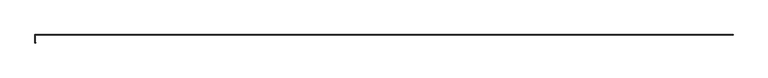
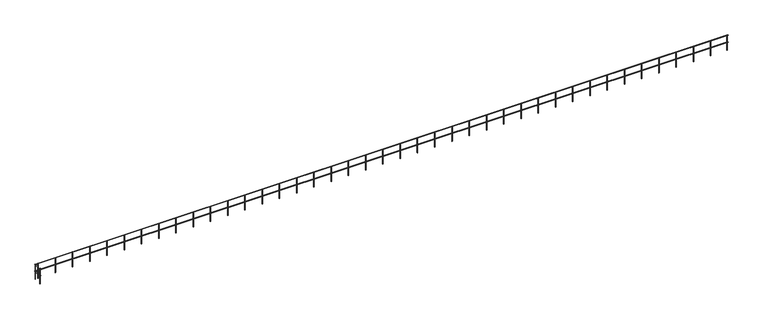
"""IFC4 building model written with IfcOpenShell, lengths in millimetres: railing geometry."""

import ifcopenshell
import ifcopenshell.guid

model = None  # the IFC model being written
_history = None  # IfcOwnerHistory: only IFC2X3 demands one
_inside = {}  # id of a spatial element -> (the spatial element, [elements in it])
_under = {}  # id of a project, library or spatial element -> (it, [spatial elements below it])
_declared = {}  # id of a project -> (the project, [libraries it declares])
_typed = {}  # id of a type object -> (the type object, [elements of that type])
_made_of = {}  # id of a material, layer set ... -> (it, [elements and type objects made of it])


def new_model(schema):
    """Start an empty IFC model of exactly this schema.

    Asked for "IFC4X3", IfcOpenShell would pick the latest addendum, in which some entities
    have other attributes; the version numbers below select the first issue.
    IFC2X3 requires an IfcOwnerHistory on every rooted entity: one is made here for all.
    """
    global model, _history
    if schema == "IFC4X3":
        model = ifcopenshell.file(schema_version=(4, 3, 0, 0))
    else:
        model = ifcopenshell.file(schema=schema)
    _inside.clear()
    _under.clear()
    _declared.clear()
    _typed.clear()
    _made_of.clear()
    _history = None
    if model.schema == "IFC2X3":
        org = make("IfcOrganization", Name="unknown")
        user = make(
            "IfcPersonAndOrganization",
            ThePerson=make("IfcPerson", FamilyName="unknown"),
            TheOrganization=org,
        )
        app = make(
            "IfcApplication",
            ApplicationDeveloper=org,
            Version="unknown",
            ApplicationFullName="unknown",
            ApplicationIdentifier="unknown",
        )
        _history = make(
            "IfcOwnerHistory",
            OwningUser=user,
            OwningApplication=app,
            ChangeAction="ADDED",
            CreationDate=0,
        )
    return model


def make(cls, **values):
    """One entity of the class cls with the attributes given. An attribute that is None is left unset."""
    return model.create_entity(
        cls, **{name: value for name, value in values.items() if value is not None}
    )


def rooted(cls, **values):
    """An entity with a GlobalId (a new one), such as an element, a storey or a relation."""
    return make(cls, GlobalId=ifcopenshell.guid.new(), OwnerHistory=_history, **values)


def si_unit(unit_type, name, prefix=None):
    """IfcSIUnit, for example si_unit("LENGTHUNIT", "METRE", prefix="MILLI")."""
    return make("IfcSIUnit", UnitType=unit_type, Prefix=prefix, Name=name)


def assignment(units):
    """IfcUnitAssignment: the units of a project."""
    return None if units is None else make("IfcUnitAssignment", Units=units)


def point(xyz):
    """IfcCartesianPoint."""
    return None if xyz is None else make("IfcCartesianPoint", Coordinates=xyz)


def direction(xyz):
    """IfcDirection."""
    return None if xyz is None else make("IfcDirection", DirectionRatios=xyz)


def frame(location, z_axis=None, x_axis=None):
    """IfcAxis2Placement3D, a coordinate frame: its origin and axes. An axis left out is left unset."""
    return make(
        "IfcAxis2Placement3D",
        Location=point(location),
        Axis=direction(z_axis),
        RefDirection=direction(x_axis),
    )


def frame_2d(location, x_axis=None):
    """IfcAxis2Placement2D, a coordinate frame in the plane: its origin and x axis."""
    return make(
        "IfcAxis2Placement2D", Location=point(location), RefDirection=direction(x_axis)
    )


def origin():
    """The frame at (0, 0, 0) with its axes left unset."""
    return frame((0.0, 0.0, 0.0))


def place(relative_to, where):
    """IfcLocalPlacement: puts the frame where relative to a parent placement (None: the world)."""
    return make(
        "IfcLocalPlacement", PlacementRelTo=relative_to, RelativePlacement=where
    )


def context(
    kind, dimensions, precision=None, world=None, true_north=None, identifier=None
):
    """IfcGeometricRepresentationContext, for example the 3D "Model" context."""
    return make(
        "IfcGeometricRepresentationContext",
        ContextIdentifier=identifier,
        ContextType=kind,
        CoordinateSpaceDimension=dimensions,
        Precision=precision,
        WorldCoordinateSystem=world,
        TrueNorth=true_north,
    )


def project(units=None, contexts=None):
    """IfcProject with its units and contexts."""
    return rooted(
        "IfcProject",
        Name="project",
        RepresentationContexts=contexts,
        UnitsInContext=assignment(units),
    )


def spatial(cls, under=None, at=None, **own):
    """A site, building, storey or space (cls), placed at a placement, below another one or the project."""
    s = rooted(cls, ObjectPlacement=at, **own)
    if under is not None:
        _under.setdefault(under.id(), (under, []))[1].append(s)
    return s


def circle_curve(where, radius):
    """IfcCircle in the frame where."""
    return make("IfcCircle", Position=where, Radius=radius)


def ellipse_curve(where, semi_axis1, semi_axis2):
    """IfcEllipse in the frame where."""
    return make(
        "IfcEllipse", Position=where, SemiAxis1=semi_axis1, SemiAxis2=semi_axis2
    )


def trimmed(basis, trim1, trim2, sense, master):
    """IfcTrimmedCurve: the piece of a basis curve between two trims."""
    return make(
        "IfcTrimmedCurve",
        BasisCurve=basis,
        Trim1=trim1,
        Trim2=trim2,
        SenseAgreement=sense,
        MasterRepresentation=master,
    )


def segment(curve, same_sense, transition):
    """IfcCompositeCurveSegment."""
    return make(
        "IfcCompositeCurveSegment",
        Transition=transition,
        SameSense=same_sense,
        ParentCurve=curve,
    )


def composite_curve(segments, self_intersect=None):
    """IfcCompositeCurve: segments joined end to end."""
    return make("IfcCompositeCurve", Segments=segments, SelfIntersect=self_intersect)


def outline(outer, holes=None, kind="AREA"):
    """IfcArbitraryClosedProfileDef: a profile drawn as a closed curve; with holes, ...WithVoids."""
    if holes is None:
        return make("IfcArbitraryClosedProfileDef", ProfileType=kind, OuterCurve=outer)
    return make(
        "IfcArbitraryProfileDefWithVoids",
        ProfileType=kind,
        OuterCurve=outer,
        InnerCurves=holes,
    )


def extrude(swept, where, along, depth):
    """IfcExtrudedAreaSolid: the profile swept, set in the frame where, extruded along a direction by depth."""
    return make(
        "IfcExtrudedAreaSolid",
        SweptArea=swept,
        Position=where,
        ExtrudedDirection=direction(along),
        Depth=depth,
    )


def shape(context_of_items, identifier, shape_type, items):
    """IfcShapeRepresentation: the items that make up one representation, for example the "Body"."""
    return make(
        "IfcShapeRepresentation",
        ContextOfItems=context_of_items,
        RepresentationIdentifier=identifier,
        RepresentationType=shape_type,
        Items=items,
    )


def source(mapping_origin, context_of_items, identifier, shape_type, items):
    """IfcRepresentationMap: a shape defined once, which mapped items show again and again."""
    return make(
        "IfcRepresentationMap",
        MappingOrigin=mapping_origin,
        MappedRepresentation=shape(context_of_items, identifier, shape_type, items),
    )


def transform(
    local_origin,
    x_axis=None,
    y_axis=None,
    z_axis=None,
    scale=None,
    scale2=None,
    scale3=None,
    uniform=True,
):
    """IfcCartesianTransformationOperator3D, or its non-uniform kind. x_axis, y_axis, z_axis: its Axis1, 2, 3."""
    if uniform:
        return make(
            "IfcCartesianTransformationOperator3D",
            Axis1=direction(x_axis),
            Axis2=direction(y_axis),
            LocalOrigin=point(local_origin),
            Scale=scale,
            Axis3=direction(z_axis),
        )
    return make(
        "IfcCartesianTransformationOperator3DnonUniform",
        Axis1=direction(x_axis),
        Axis2=direction(y_axis),
        LocalOrigin=point(local_origin),
        Scale=scale,
        Axis3=direction(z_axis),
        Scale2=scale2,
        Scale3=scale3,
    )


def mapped(mapping_source, mapping_target):
    """IfcMappedItem: shows the shape of a source again, moved by a transform."""
    return make(
        "IfcMappedItem", MappingSource=mapping_source, MappingTarget=mapping_target
    )


def made_of(thing, what):
    """Note that an element or type object is made of a material, layer set ...; save() writes the relation."""
    if what is not None:
        _made_of.setdefault(what.id(), (what, []))[1].append(thing)
    return thing


def element(
    cls,
    number,
    at=None,
    inside=None,
    cuts=None,
    type_object=None,
    material=None,
    context=None,
    identifier="Body",
    shape_type=None,
    held_by="IfcProductDefinitionShape",
    body=None,
    shapes=None,
    **own,
):
    """One element of the class cls, such as IfcWall. Its Tag is "e" and its number.

    at: its placement. inside: the storey or other place that contains it. cuts: it is an
    opening in that element (IfcRelVoidsElement). A single representation is given by context,
    identifier, shape_type and body (its items); several are given by shapes. held_by: the class
    of the entity that holds the representations. save() writes the other relations.
    """
    e = rooted(cls, Tag="e%d" % number, ObjectPlacement=at, **own)
    if body is not None:
        shapes = [shape(context, identifier, shape_type, body)]
    if shapes is not None:
        e.Representation = make(held_by, Representations=shapes)
    if inside is not None:
        _inside.setdefault(inside.id(), (inside, []))[1].append(e)
    if cuts is not None:
        rooted(
            "IfcRelVoidsElement", RelatingBuildingElement=cuts, RelatedOpeningElement=e
        )
    if type_object is not None:
        _typed.setdefault(type_object.id(), (type_object, []))[1].append(e)
    return made_of(e, material)


def aggregate(whole, parts):
    """IfcRelAggregates: a whole, such as a stair, and the parts it consists of."""
    return rooted("IfcRelAggregates", RelatingObject=whole, RelatedObjects=parts)


def save(model, path):
    """Write the relations noted so far, then the file.

    IfcRelAggregates (storeys below a building ...), IfcRelContainedInSpatialStructure (elements
    in a storey), IfcRelDefinesByType, IfcRelAssociatesMaterial and IfcRelDeclares: one each for
    every whole, place, type object, material and project.
    """
    for whole, parts in _under.values():
        aggregate(whole, parts)
    for where, things in _inside.values():
        rooted(
            "IfcRelContainedInSpatialStructure",
            RelatedElements=things,
            RelatingStructure=where,
        )
    for kind, things in _typed.values():
        rooted("IfcRelDefinesByType", RelatedObjects=things, RelatingType=kind)
    for what, things in _made_of.values():
        rooted("IfcRelAssociatesMaterial", RelatedObjects=things, RelatingMaterial=what)
    for by, libraries in _declared.values():
        rooted("IfcRelDeclares", RelatingContext=by, RelatedDefinitions=libraries)
    model.write(path)


def plane_surface(at):
    """IfcPlane: the flat surface through the origin of the frame at, square to its z axis."""
    return make("IfcPlane", Position=at)


def cylinder_surface(at, radius):
    """IfcCylindricalSurface: all points at the distance radius from the z axis of the frame at."""
    return make("IfcCylindricalSurface", Position=at, Radius=radius)


def advanced_brep(points, edges, surfaces, faces):
    """IfcAdvancedBrep: a solid bounded by faces that lie on surfaces and meet in shared edges.

    An edge is (start, end): straight between two places in points (the first is 0);
    or (start, end, curve); or (start, end, curve, False) where it runs against its curve.
    A face is (place in surfaces, loops), or (place, loops, False) where it looks against
    its surface's normal. A loop lists edges by number (the first is 1), with a minus sign
    where the edge is run from its end to its start. The first loop is the outer one.
    """
    corners = [point(p) for p in points]
    vertices = [make("IfcVertexPoint", VertexGeometry=c) for c in corners]
    made = []
    for start, end, *more in edges:
        made.append(
            make(
                "IfcEdgeCurve",
                EdgeStart=vertices[start],
                EdgeEnd=vertices[end],
                EdgeGeometry=more[0] if more else make("IfcPolyline", Points=[corners[start], corners[end]]),
                SameSense=more[1] if len(more) > 1 else True,
            )
        )
    hull = []
    for where, loops, *sense in faces:
        bounds = []
        for j, loop in enumerate(loops):
            ring = [make("IfcOrientedEdge", EdgeElement=made[abs(k) - 1], Orientation=k > 0) for k in loop]
            bounds.append(
                make(
                    "IfcFaceOuterBound" if j == 0 else "IfcFaceBound",
                    Bound=make("IfcEdgeLoop", EdgeList=ring),
                    Orientation=True,
                )
            )
        hull.append(make("IfcAdvancedFace", Bounds=bounds, FaceSurface=surfaces[where], SameSense=sense[0] if sense else True))
    return make("IfcAdvancedBrep", Outer=make("IfcClosedShell", CfsFaces=hull))


def railing_e0085468(model_context):
    return source(origin(), model_context, "Body", "SolidModel", [
        advanced_brep(
        [(74181.0, -4167.9791411, 885.0), (74181.0, -4137.9791411, 885.0), (26002.0, -4167.9791411, 885.0), (25972.0, -4137.9791411, 885.0), (26002.0, -4687.9791411, 885.0), (25972.0, -4717.9791411, 885.0), (26040.0, -4687.9791411, 885.0), (26040.0, -4717.9791411, 885.0)],
        [
            (0, 1, circle_curve(frame((74181.0, -4152.9791411, 885.0), z_axis=(1.0, 0.0, 0.0), x_axis=(0.0, 1.0, 0.0)), 15.0)),
            (1, 0, circle_curve(frame((74181.0, -4152.9791411, 885.0), z_axis=(1.0, 0.0, 0.0), x_axis=(0.0, 1.0, 0.0)), 15.0)),
            (0, 2),
            (2, 3, ellipse_curve(frame((25987.0, -4152.9791411, 885.0), z_axis=(0.7071067811865487, 0.7071067811865464, 0.0), x_axis=(0.7071067811865465, -0.7071067811865487, 0.0)), 21.2132034, 15.0)),
            (3, 1),
            (3, 2, ellipse_curve(frame((25987.0, -4152.9791411, 885.0), z_axis=(0.7071067811865487, 0.7071067811865464, 0.0), x_axis=(0.7071067811865465, -0.7071067811865487, 0.0)), 21.2132034, 15.0)),
            (2, 4),
            (4, 5, ellipse_curve(frame((25987.0, -4702.9791411, 885.0), z_axis=(-0.7071067811865475, 0.7071067811865475, 0.0), x_axis=(0.7071067811865474, 0.7071067811865476, 0.0)), 21.2132034, 15.0)),
            (5, 3),
            (5, 4, ellipse_curve(frame((25987.0, -4702.9791411, 885.0), z_axis=(-0.7071067811865475, 0.7071067811865475, 0.0), x_axis=(0.7071067811865474, 0.7071067811865476, 0.0)), 21.2132034, 15.0)),
            (6, 7, circle_curve(frame((26040.0, -4702.9791411, 885.0), z_axis=(1.0, 0.0, 0.0), x_axis=(0.0, -1.0, 0.0)), 15.0)),
            (7, 6, circle_curve(frame((26040.0, -4702.9791411, 885.0), z_axis=(1.0, 0.0, 0.0), x_axis=(0.0, -1.0, 0.0)), 15.0)),
            (4, 6),
            (7, 5),
        ],
        [
            plane_surface(frame((74181.0, -4152.9791411, 900.0), z_axis=(1.0, 0.0, 0.0), x_axis=(0.0, -1.0, 0.0))),
            cylinder_surface(frame((74181.0, -4152.9791411, 885.0), z_axis=(1.0, 0.0, 0.0), x_axis=(0.0, 1.0, 0.0)), 15.0),
            cylinder_surface(frame((25987.0, -4152.9791411, 885.0), z_axis=(0.0, 1.0, 0.0), x_axis=(-1.0, 0.0, 0.0)), 15.0),
            plane_surface(frame((26040.0, -4702.9791411, 900.0), z_axis=(1.0, 0.0, 0.0), x_axis=(0.0, 1.0, 0.0))),
            cylinder_surface(frame((25987.0, -4702.9791411, 885.0), z_axis=(-1.0, 0.0, 0.0), x_axis=(0.0, -1.0, 0.0)), 15.0),
        ],
        [
            (0, [[1, 2]]),
            (1, [[-1, 3, 4, 5]]),
            (1, [[-2, -5, 6, -3]]),
            (2, [[-4, 7, 8, 9]]),
            (2, [[-6, -9, 10, -7]]),
            (3, [[11, 12]]),
            (4, [[-8, 13, -12, 14]]),
            (4, [[-10, -14, -11, -13]]),
        ],
    ),
        advanced_brep(
        [(74181.0, -4167.9791411, 1385.0), (74181.0, -4137.9791411, 1385.0), (26002.0, -4167.9791411, 1385.0), (25972.0, -4137.9791411, 1385.0), (26002.0, -4687.9791411, 1385.0), (25972.0, -4717.9791411, 1385.0), (26040.0, -4687.9791411, 1385.0), (26040.0, -4717.9791411, 1385.0)],
        [
            (0, 1, circle_curve(frame((74181.0, -4152.9791411, 1385.0), z_axis=(1.0, 0.0, 0.0), x_axis=(0.0, 1.0, 0.0)), 15.0)),
            (1, 0, circle_curve(frame((74181.0, -4152.9791411, 1385.0), z_axis=(1.0, 0.0, 0.0), x_axis=(0.0, 1.0, 0.0)), 15.0)),
            (0, 2),
            (2, 3, ellipse_curve(frame((25987.0, -4152.9791411, 1385.0), z_axis=(0.7071067811865487, 0.7071067811865464, 0.0), x_axis=(0.7071067811865465, -0.7071067811865487, 0.0)), 21.2132034, 15.0)),
            (3, 1),
            (3, 2, ellipse_curve(frame((25987.0, -4152.9791411, 1385.0), z_axis=(0.7071067811865487, 0.7071067811865464, 0.0), x_axis=(0.7071067811865465, -0.7071067811865487, 0.0)), 21.2132034, 15.0)),
            (2, 4),
            (4, 5, ellipse_curve(frame((25987.0, -4702.9791411, 1385.0), z_axis=(-0.7071067811865475, 0.7071067811865475, 0.0), x_axis=(0.7071067811865474, 0.7071067811865476, 0.0)), 21.2132034, 15.0)),
            (5, 3),
            (5, 4, ellipse_curve(frame((25987.0, -4702.9791411, 1385.0), z_axis=(-0.7071067811865475, 0.7071067811865475, 0.0), x_axis=(0.7071067811865474, 0.7071067811865476, 0.0)), 21.2132034, 15.0)),
            (6, 7, circle_curve(frame((26040.0, -4702.9791411, 1385.0), z_axis=(1.0, 0.0, 0.0), x_axis=(0.0, -1.0, 0.0)), 15.0)),
            (7, 6, circle_curve(frame((26040.0, -4702.9791411, 1385.0), z_axis=(1.0, 0.0, 0.0), x_axis=(0.0, -1.0, 0.0)), 15.0)),
            (4, 6),
            (7, 5),
        ],
        [
            plane_surface(frame((74181.0, -4152.9791411, 1400.0), z_axis=(1.0, 0.0, 0.0), x_axis=(0.0, -1.0, 0.0))),
            cylinder_surface(frame((74181.0, -4152.9791411, 1385.0), z_axis=(1.0, 0.0, 0.0), x_axis=(0.0, 1.0, 0.0)), 15.0),
            cylinder_surface(frame((25987.0, -4152.9791411, 1385.0), z_axis=(0.0, 1.0, 0.0), x_axis=(-1.0, 0.0, 0.0)), 15.0),
            plane_surface(frame((26040.0, -4702.9791411, 1400.0), z_axis=(1.0, 0.0, 0.0), x_axis=(0.0, 1.0, 0.0))),
            cylinder_surface(frame((25987.0, -4702.9791411, 1385.0), z_axis=(-1.0, 0.0, 0.0), x_axis=(0.0, -1.0, 0.0)), 15.0),
        ],
        [
            (0, [[1, 2]]),
            (1, [[-1, 3, 4, 5]]),
            (1, [[-2, -5, 6, -3]]),
            (2, [[-4, 7, 8, 9]]),
            (2, [[-6, -9, 10, -7]]),
            (3, [[11, 12]]),
            (4, [[-8, 13, -12, 14]]),
            (4, [[-10, -14, -11, -13]]),
        ],
    ),
        extrude(outline(composite_curve([segment(trimmed(circle_curve(frame_2d((26181.0, -4152.9791411)), 15.0), [point((26181.0, -4167.9791411))], [point((26181.0, -4137.9791411))], False, "CARTESIAN"), True, "CONTINUOUS"), segment(trimmed(circle_curve(frame_2d((26181.0, -4152.9791411)), 15.0), [point((26181.0, -4137.9791411))], [point((26181.0, -4167.9791411))], False, "CARTESIAN"), True, "CONTINUOUS")], self_intersect=False)), frame((0.0, 0.0, 300.0), z_axis=(0.0, 0.0, 1.0), x_axis=(1.0, 0.0, 0.0)), (0.0, 0.0, 1.0), 1070.0),
        extrude(outline(composite_curve([segment(trimmed(circle_curve(frame_2d((27381.0, -4152.9791411)), 15.0), [point((27381.0, -4167.9791411))], [point((27381.0, -4137.9791411))], False, "CARTESIAN"), True, "CONTINUOUS"), segment(trimmed(circle_curve(frame_2d((27381.0, -4152.9791411)), 15.0), [point((27381.0, -4137.9791411))], [point((27381.0, -4167.9791411))], False, "CARTESIAN"), True, "CONTINUOUS")], self_intersect=False)), frame((0.0, 0.0, 300.0), z_axis=(0.0, 0.0, 1.0), x_axis=(1.0, 0.0, 0.0)), (0.0, 0.0, 1.0), 1070.0),
        extrude(outline(composite_curve([segment(trimmed(circle_curve(frame_2d((28581.0, -4152.9791411)), 15.0), [point((28581.0, -4167.9791411))], [point((28581.0, -4137.9791411))], False, "CARTESIAN"), True, "CONTINUOUS"), segment(trimmed(circle_curve(frame_2d((28581.0, -4152.9791411)), 15.0), [point((28581.0, -4137.9791411))], [point((28581.0, -4167.9791411))], False, "CARTESIAN"), True, "CONTINUOUS")], self_intersect=False)), frame((0.0, 0.0, 300.0), z_axis=(0.0, 0.0, 1.0), x_axis=(1.0, 0.0, 0.0)), (0.0, 0.0, 1.0), 1070.0),
        extrude(outline(composite_curve([segment(trimmed(circle_curve(frame_2d((29781.0, -4152.9791411)), 15.0), [point((29781.0, -4167.9791411))], [point((29781.0, -4137.9791411))], False, "CARTESIAN"), True, "CONTINUOUS"), segment(trimmed(circle_curve(frame_2d((29781.0, -4152.9791411)), 15.0), [point((29781.0, -4137.9791411))], [point((29781.0, -4167.9791411))], False, "CARTESIAN"), True, "CONTINUOUS")], self_intersect=False)), frame((0.0, 0.0, 300.0), z_axis=(0.0, 0.0, 1.0), x_axis=(1.0, 0.0, 0.0)), (0.0, 0.0, 1.0), 1070.0),
        extrude(outline(composite_curve([segment(trimmed(circle_curve(frame_2d((30981.0, -4152.9791411)), 15.0), [point((30981.0, -4167.9791411))], [point((30981.0, -4137.9791411))], False, "CARTESIAN"), True, "CONTINUOUS"), segment(trimmed(circle_curve(frame_2d((30981.0, -4152.9791411)), 15.0), [point((30981.0, -4137.9791411))], [point((30981.0, -4167.9791411))], False, "CARTESIAN"), True, "CONTINUOUS")], self_intersect=False)), frame((0.0, 0.0, 300.0), z_axis=(0.0, 0.0, 1.0), x_axis=(1.0, 0.0, 0.0)), (0.0, 0.0, 1.0), 1070.0),
        extrude(outline(composite_curve([segment(trimmed(circle_curve(frame_2d((32181.0, -4152.9791411)), 15.0), [point((32181.0, -4167.9791411))], [point((32181.0, -4137.9791411))], False, "CARTESIAN"), True, "CONTINUOUS"), segment(trimmed(circle_curve(frame_2d((32181.0, -4152.9791411)), 15.0), [point((32181.0, -4137.9791411))], [point((32181.0, -4167.9791411))], False, "CARTESIAN"), True, "CONTINUOUS")], self_intersect=False)), frame((0.0, 0.0, 300.0), z_axis=(0.0, 0.0, 1.0), x_axis=(1.0, 0.0, 0.0)), (0.0, 0.0, 1.0), 1070.0),
        extrude(outline(composite_curve([segment(trimmed(circle_curve(frame_2d((33381.0, -4152.9791411)), 15.0), [point((33381.0, -4167.9791411))], [point((33381.0, -4137.9791411))], False, "CARTESIAN"), True, "CONTINUOUS"), segment(trimmed(circle_curve(frame_2d((33381.0, -4152.9791411)), 15.0), [point((33381.0, -4137.9791411))], [point((33381.0, -4167.9791411))], False, "CARTESIAN"), True, "CONTINUOUS")], self_intersect=False)), frame((0.0, 0.0, 300.0), z_axis=(0.0, 0.0, 1.0), x_axis=(1.0, 0.0, 0.0)), (0.0, 0.0, 1.0), 1070.0),
        extrude(outline(composite_curve([segment(trimmed(circle_curve(frame_2d((34581.0, -4152.9791411)), 15.0), [point((34581.0, -4167.9791411))], [point((34581.0, -4137.9791411))], False, "CARTESIAN"), True, "CONTINUOUS"), segment(trimmed(circle_curve(frame_2d((34581.0, -4152.9791411)), 15.0), [point((34581.0, -4137.9791411))], [point((34581.0, -4167.9791411))], False, "CARTESIAN"), True, "CONTINUOUS")], self_intersect=False)), frame((0.0, 0.0, 300.0), z_axis=(0.0, 0.0, 1.0), x_axis=(1.0, 0.0, 0.0)), (0.0, 0.0, 1.0), 1070.0),
        extrude(outline(composite_curve([segment(trimmed(circle_curve(frame_2d((35781.0, -4152.9791411)), 15.0), [point((35781.0, -4167.9791411))], [point((35781.0, -4137.9791411))], False, "CARTESIAN"), True, "CONTINUOUS"), segment(trimmed(circle_curve(frame_2d((35781.0, -4152.9791411)), 15.0), [point((35781.0, -4137.9791411))], [point((35781.0, -4167.9791411))], False, "CARTESIAN"), True, "CONTINUOUS")], self_intersect=False)), frame((0.0, 0.0, 300.0), z_axis=(0.0, 0.0, 1.0), x_axis=(1.0, 0.0, 0.0)), (0.0, 0.0, 1.0), 1070.0),
        extrude(outline(composite_curve([segment(trimmed(circle_curve(frame_2d((36981.0, -4152.9791411)), 15.0), [point((36981.0, -4167.9791411))], [point((36981.0, -4137.9791411))], False, "CARTESIAN"), True, "CONTINUOUS"), segment(trimmed(circle_curve(frame_2d((36981.0, -4152.9791411)), 15.0), [point((36981.0, -4137.9791411))], [point((36981.0, -4167.9791411))], False, "CARTESIAN"), True, "CONTINUOUS")], self_intersect=False)), frame((0.0, 0.0, 300.0), z_axis=(0.0, 0.0, 1.0), x_axis=(1.0, 0.0, 0.0)), (0.0, 0.0, 1.0), 1070.0),
        extrude(outline(composite_curve([segment(trimmed(circle_curve(frame_2d((38181.0, -4152.9791411)), 15.0), [point((38181.0, -4167.9791411))], [point((38181.0, -4137.9791411))], False, "CARTESIAN"), True, "CONTINUOUS"), segment(trimmed(circle_curve(frame_2d((38181.0, -4152.9791411)), 15.0), [point((38181.0, -4137.9791411))], [point((38181.0, -4167.9791411))], False, "CARTESIAN"), True, "CONTINUOUS")], self_intersect=False)), frame((0.0, 0.0, 300.0), z_axis=(0.0, 0.0, 1.0), x_axis=(1.0, 0.0, 0.0)), (0.0, 0.0, 1.0), 1070.0),
        extrude(outline(composite_curve([segment(trimmed(circle_curve(frame_2d((39381.0, -4152.9791411)), 15.0), [point((39381.0, -4167.9791411))], [point((39381.0, -4137.9791411))], False, "CARTESIAN"), True, "CONTINUOUS"), segment(trimmed(circle_curve(frame_2d((39381.0, -4152.9791411)), 15.0), [point((39381.0, -4137.9791411))], [point((39381.0, -4167.9791411))], False, "CARTESIAN"), True, "CONTINUOUS")], self_intersect=False)), frame((0.0, 0.0, 300.0), z_axis=(0.0, 0.0, 1.0), x_axis=(1.0, 0.0, 0.0)), (0.0, 0.0, 1.0), 1070.0),
        extrude(outline(composite_curve([segment(trimmed(circle_curve(frame_2d((40581.0, -4152.9791411)), 15.0), [point((40581.0, -4167.9791411))], [point((40581.0, -4137.9791411))], False, "CARTESIAN"), True, "CONTINUOUS"), segment(trimmed(circle_curve(frame_2d((40581.0, -4152.9791411)), 15.0), [point((40581.0, -4137.9791411))], [point((40581.0, -4167.9791411))], False, "CARTESIAN"), True, "CONTINUOUS")], self_intersect=False)), frame((0.0, 0.0, 300.0), z_axis=(0.0, 0.0, 1.0), x_axis=(1.0, 0.0, 0.0)), (0.0, 0.0, 1.0), 1070.0),
        extrude(outline(composite_curve([segment(trimmed(circle_curve(frame_2d((41781.0, -4152.9791411)), 15.0), [point((41781.0, -4167.9791411))], [point((41781.0, -4137.9791411))], False, "CARTESIAN"), True, "CONTINUOUS"), segment(trimmed(circle_curve(frame_2d((41781.0, -4152.9791411)), 15.0), [point((41781.0, -4137.9791411))], [point((41781.0, -4167.9791411))], False, "CARTESIAN"), True, "CONTINUOUS")], self_intersect=False)), frame((0.0, 0.0, 300.0), z_axis=(0.0, 0.0, 1.0), x_axis=(1.0, 0.0, 0.0)), (0.0, 0.0, 1.0), 1070.0),
        extrude(outline(composite_curve([segment(trimmed(circle_curve(frame_2d((42981.0, -4152.9791411)), 15.0), [point((42981.0, -4167.9791411))], [point((42981.0, -4137.9791411))], False, "CARTESIAN"), True, "CONTINUOUS"), segment(trimmed(circle_curve(frame_2d((42981.0, -4152.9791411)), 15.0), [point((42981.0, -4137.9791411))], [point((42981.0, -4167.9791411))], False, "CARTESIAN"), True, "CONTINUOUS")], self_intersect=False)), frame((0.0, 0.0, 300.0), z_axis=(0.0, 0.0, 1.0), x_axis=(1.0, 0.0, 0.0)), (0.0, 0.0, 1.0), 1070.0),
        extrude(outline(composite_curve([segment(trimmed(circle_curve(frame_2d((44181.0, -4152.9791411)), 15.0), [point((44181.0, -4167.9791411))], [point((44181.0, -4137.9791411))], False, "CARTESIAN"), True, "CONTINUOUS"), segment(trimmed(circle_curve(frame_2d((44181.0, -4152.9791411)), 15.0), [point((44181.0, -4137.9791411))], [point((44181.0, -4167.9791411))], False, "CARTESIAN"), True, "CONTINUOUS")], self_intersect=False)), frame((0.0, 0.0, 300.0), z_axis=(0.0, 0.0, 1.0), x_axis=(1.0, 0.0, 0.0)), (0.0, 0.0, 1.0), 1070.0),
        extrude(outline(composite_curve([segment(trimmed(circle_curve(frame_2d((45381.0, -4152.9791411)), 15.0), [point((45381.0, -4167.9791411))], [point((45381.0, -4137.9791411))], False, "CARTESIAN"), True, "CONTINUOUS"), segment(trimmed(circle_curve(frame_2d((45381.0, -4152.9791411)), 15.0), [point((45381.0, -4137.9791411))], [point((45381.0, -4167.9791411))], False, "CARTESIAN"), True, "CONTINUOUS")], self_intersect=False)), frame((0.0, 0.0, 300.0), z_axis=(0.0, 0.0, 1.0), x_axis=(1.0, 0.0, 0.0)), (0.0, 0.0, 1.0), 1070.0),
        extrude(outline(composite_curve([segment(trimmed(circle_curve(frame_2d((46581.0, -4152.9791411)), 15.0), [point((46581.0, -4167.9791411))], [point((46581.0, -4137.9791411))], False, "CARTESIAN"), True, "CONTINUOUS"), segment(trimmed(circle_curve(frame_2d((46581.0, -4152.9791411)), 15.0), [point((46581.0, -4137.9791411))], [point((46581.0, -4167.9791411))], False, "CARTESIAN"), True, "CONTINUOUS")], self_intersect=False)), frame((0.0, 0.0, 300.0), z_axis=(0.0, 0.0, 1.0), x_axis=(1.0, 0.0, 0.0)), (0.0, 0.0, 1.0), 1070.0),
        extrude(outline(composite_curve([segment(trimmed(circle_curve(frame_2d((47781.0, -4152.9791411)), 15.0), [point((47781.0, -4167.9791411))], [point((47781.0, -4137.9791411))], False, "CARTESIAN"), True, "CONTINUOUS"), segment(trimmed(circle_curve(frame_2d((47781.0, -4152.9791411)), 15.0), [point((47781.0, -4137.9791411))], [point((47781.0, -4167.9791411))], False, "CARTESIAN"), True, "CONTINUOUS")], self_intersect=False)), frame((0.0, 0.0, 300.0), z_axis=(0.0, 0.0, 1.0), x_axis=(1.0, 0.0, 0.0)), (0.0, 0.0, 1.0), 1070.0),
        extrude(outline(composite_curve([segment(trimmed(circle_curve(frame_2d((48981.0, -4152.9791411)), 15.0), [point((48981.0, -4167.9791411))], [point((48981.0, -4137.9791411))], False, "CARTESIAN"), True, "CONTINUOUS"), segment(trimmed(circle_curve(frame_2d((48981.0, -4152.9791411)), 15.0), [point((48981.0, -4137.9791411))], [point((48981.0, -4167.9791411))], False, "CARTESIAN"), True, "CONTINUOUS")], self_intersect=False)), frame((0.0, 0.0, 300.0), z_axis=(0.0, 0.0, 1.0), x_axis=(1.0, 0.0, 0.0)), (0.0, 0.0, 1.0), 1070.0),
        extrude(outline(composite_curve([segment(trimmed(circle_curve(frame_2d((50181.0, -4152.9791411)), 15.0), [point((50181.0, -4167.9791411))], [point((50181.0, -4137.9791411))], False, "CARTESIAN"), True, "CONTINUOUS"), segment(trimmed(circle_curve(frame_2d((50181.0, -4152.9791411)), 15.0), [point((50181.0, -4137.9791411))], [point((50181.0, -4167.9791411))], False, "CARTESIAN"), True, "CONTINUOUS")], self_intersect=False)), frame((0.0, 0.0, 300.0), z_axis=(0.0, 0.0, 1.0), x_axis=(1.0, 0.0, 0.0)), (0.0, 0.0, 1.0), 1070.0),
        extrude(outline(composite_curve([segment(trimmed(circle_curve(frame_2d((51381.0, -4152.9791411)), 15.0), [point((51381.0, -4167.9791411))], [point((51381.0, -4137.9791411))], False, "CARTESIAN"), True, "CONTINUOUS"), segment(trimmed(circle_curve(frame_2d((51381.0, -4152.9791411)), 15.0), [point((51381.0, -4137.9791411))], [point((51381.0, -4167.9791411))], False, "CARTESIAN"), True, "CONTINUOUS")], self_intersect=False)), frame((0.0, 0.0, 300.0), z_axis=(0.0, 0.0, 1.0), x_axis=(1.0, 0.0, 0.0)), (0.0, 0.0, 1.0), 1070.0),
        extrude(outline(composite_curve([segment(trimmed(circle_curve(frame_2d((52581.0, -4152.9791411)), 15.0), [point((52581.0, -4167.9791411))], [point((52581.0, -4137.9791411))], False, "CARTESIAN"), True, "CONTINUOUS"), segment(trimmed(circle_curve(frame_2d((52581.0, -4152.9791411)), 15.0), [point((52581.0, -4137.9791411))], [point((52581.0, -4167.9791411))], False, "CARTESIAN"), True, "CONTINUOUS")], self_intersect=False)), frame((0.0, 0.0, 300.0), z_axis=(0.0, 0.0, 1.0), x_axis=(1.0, 0.0, 0.0)), (0.0, 0.0, 1.0), 1070.0),
        extrude(outline(composite_curve([segment(trimmed(circle_curve(frame_2d((53781.0, -4152.9791411)), 15.0), [point((53781.0, -4167.9791411))], [point((53781.0, -4137.9791411))], False, "CARTESIAN"), True, "CONTINUOUS"), segment(trimmed(circle_curve(frame_2d((53781.0, -4152.9791411)), 15.0), [point((53781.0, -4137.9791411))], [point((53781.0, -4167.9791411))], False, "CARTESIAN"), True, "CONTINUOUS")], self_intersect=False)), frame((0.0, 0.0, 300.0), z_axis=(0.0, 0.0, 1.0), x_axis=(1.0, 0.0, 0.0)), (0.0, 0.0, 1.0), 1070.0),
        extrude(outline(composite_curve([segment(trimmed(circle_curve(frame_2d((54981.0, -4152.9791411)), 15.0), [point((54981.0, -4167.9791411))], [point((54981.0, -4137.9791411))], False, "CARTESIAN"), True, "CONTINUOUS"), segment(trimmed(circle_curve(frame_2d((54981.0, -4152.9791411)), 15.0), [point((54981.0, -4137.9791411))], [point((54981.0, -4167.9791411))], False, "CARTESIAN"), True, "CONTINUOUS")], self_intersect=False)), frame((0.0, 0.0, 300.0), z_axis=(0.0, 0.0, 1.0), x_axis=(1.0, 0.0, 0.0)), (0.0, 0.0, 1.0), 1070.0),
        extrude(outline(composite_curve([segment(trimmed(circle_curve(frame_2d((56181.0, -4152.9791411)), 15.0), [point((56181.0, -4167.9791411))], [point((56181.0, -4137.9791411))], False, "CARTESIAN"), True, "CONTINUOUS"), segment(trimmed(circle_curve(frame_2d((56181.0, -4152.9791411)), 15.0), [point((56181.0, -4137.9791411))], [point((56181.0, -4167.9791411))], False, "CARTESIAN"), True, "CONTINUOUS")], self_intersect=False)), frame((0.0, 0.0, 300.0), z_axis=(0.0, 0.0, 1.0), x_axis=(1.0, 0.0, 0.0)), (0.0, 0.0, 1.0), 1070.0),
        extrude(outline(composite_curve([segment(trimmed(circle_curve(frame_2d((57381.0, -4152.9791411)), 15.0), [point((57381.0, -4167.9791411))], [point((57381.0, -4137.9791411))], False, "CARTESIAN"), True, "CONTINUOUS"), segment(trimmed(circle_curve(frame_2d((57381.0, -4152.9791411)), 15.0), [point((57381.0, -4137.9791411))], [point((57381.0, -4167.9791411))], False, "CARTESIAN"), True, "CONTINUOUS")], self_intersect=False)), frame((0.0, 0.0, 300.0), z_axis=(0.0, 0.0, 1.0), x_axis=(1.0, 0.0, 0.0)), (0.0, 0.0, 1.0), 1070.0),
        extrude(outline(composite_curve([segment(trimmed(circle_curve(frame_2d((58581.0, -4152.9791411)), 15.0), [point((58581.0, -4167.9791411))], [point((58581.0, -4137.9791411))], False, "CARTESIAN"), True, "CONTINUOUS"), segment(trimmed(circle_curve(frame_2d((58581.0, -4152.9791411)), 15.0), [point((58581.0, -4137.9791411))], [point((58581.0, -4167.9791411))], False, "CARTESIAN"), True, "CONTINUOUS")], self_intersect=False)), frame((0.0, 0.0, 300.0), z_axis=(0.0, 0.0, 1.0), x_axis=(1.0, 0.0, 0.0)), (0.0, 0.0, 1.0), 1070.0),
        extrude(outline(composite_curve([segment(trimmed(circle_curve(frame_2d((59781.0, -4152.9791411)), 15.0), [point((59781.0, -4167.9791411))], [point((59781.0, -4137.9791411))], False, "CARTESIAN"), True, "CONTINUOUS"), segment(trimmed(circle_curve(frame_2d((59781.0, -4152.9791411)), 15.0), [point((59781.0, -4137.9791411))], [point((59781.0, -4167.9791411))], False, "CARTESIAN"), True, "CONTINUOUS")], self_intersect=False)), frame((0.0, 0.0, 300.0), z_axis=(0.0, 0.0, 1.0), x_axis=(1.0, 0.0, 0.0)), (0.0, 0.0, 1.0), 1070.0),
        extrude(outline(composite_curve([segment(trimmed(circle_curve(frame_2d((60981.0, -4152.9791411)), 15.0), [point((60981.0, -4167.9791411))], [point((60981.0, -4137.9791411))], False, "CARTESIAN"), True, "CONTINUOUS"), segment(trimmed(circle_curve(frame_2d((60981.0, -4152.9791411)), 15.0), [point((60981.0, -4137.9791411))], [point((60981.0, -4167.9791411))], False, "CARTESIAN"), True, "CONTINUOUS")], self_intersect=False)), frame((0.0, 0.0, 300.0), z_axis=(0.0, 0.0, 1.0), x_axis=(1.0, 0.0, 0.0)), (0.0, 0.0, 1.0), 1070.0),
        extrude(outline(composite_curve([segment(trimmed(circle_curve(frame_2d((62181.0, -4152.9791411)), 15.0), [point((62181.0, -4167.9791411))], [point((62181.0, -4137.9791411))], False, "CARTESIAN"), True, "CONTINUOUS"), segment(trimmed(circle_curve(frame_2d((62181.0, -4152.9791411)), 15.0), [point((62181.0, -4137.9791411))], [point((62181.0, -4167.9791411))], False, "CARTESIAN"), True, "CONTINUOUS")], self_intersect=False)), frame((0.0, 0.0, 300.0), z_axis=(0.0, 0.0, 1.0), x_axis=(1.0, 0.0, 0.0)), (0.0, 0.0, 1.0), 1070.0),
        extrude(outline(composite_curve([segment(trimmed(circle_curve(frame_2d((63381.0, -4152.9791411)), 15.0), [point((63381.0, -4167.9791411))], [point((63381.0, -4137.9791411))], False, "CARTESIAN"), True, "CONTINUOUS"), segment(trimmed(circle_curve(frame_2d((63381.0, -4152.9791411)), 15.0), [point((63381.0, -4137.9791411))], [point((63381.0, -4167.9791411))], False, "CARTESIAN"), True, "CONTINUOUS")], self_intersect=False)), frame((0.0, 0.0, 300.0), z_axis=(0.0, 0.0, 1.0), x_axis=(1.0, 0.0, 0.0)), (0.0, 0.0, 1.0), 1070.0),
        extrude(outline(composite_curve([segment(trimmed(circle_curve(frame_2d((64581.0, -4152.9791411)), 15.0), [point((64581.0, -4167.9791411))], [point((64581.0, -4137.9791411))], False, "CARTESIAN"), True, "CONTINUOUS"), segment(trimmed(circle_curve(frame_2d((64581.0, -4152.9791411)), 15.0), [point((64581.0, -4137.9791411))], [point((64581.0, -4167.9791411))], False, "CARTESIAN"), True, "CONTINUOUS")], self_intersect=False)), frame((0.0, 0.0, 300.0), z_axis=(0.0, 0.0, 1.0), x_axis=(1.0, 0.0, 0.0)), (0.0, 0.0, 1.0), 1070.0),
        extrude(outline(composite_curve([segment(trimmed(circle_curve(frame_2d((65781.0, -4152.9791411)), 15.0), [point((65781.0, -4167.9791411))], [point((65781.0, -4137.9791411))], False, "CARTESIAN"), True, "CONTINUOUS"), segment(trimmed(circle_curve(frame_2d((65781.0, -4152.9791411)), 15.0), [point((65781.0, -4137.9791411))], [point((65781.0, -4167.9791411))], False, "CARTESIAN"), True, "CONTINUOUS")], self_intersect=False)), frame((0.0, 0.0, 300.0), z_axis=(0.0, 0.0, 1.0), x_axis=(1.0, 0.0, 0.0)), (0.0, 0.0, 1.0), 1070.0),
        extrude(outline(composite_curve([segment(trimmed(circle_curve(frame_2d((66981.0, -4152.9791411)), 15.0), [point((66981.0, -4167.9791411))], [point((66981.0, -4137.9791411))], False, "CARTESIAN"), True, "CONTINUOUS"), segment(trimmed(circle_curve(frame_2d((66981.0, -4152.9791411)), 15.0), [point((66981.0, -4137.9791411))], [point((66981.0, -4167.9791411))], False, "CARTESIAN"), True, "CONTINUOUS")], self_intersect=False)), frame((0.0, 0.0, 300.0), z_axis=(0.0, 0.0, 1.0), x_axis=(1.0, 0.0, 0.0)), (0.0, 0.0, 1.0), 1070.0),
        extrude(outline(composite_curve([segment(trimmed(circle_curve(frame_2d((68181.0, -4152.9791411)), 15.0), [point((68181.0, -4167.9791411))], [point((68181.0, -4137.9791411))], False, "CARTESIAN"), True, "CONTINUOUS"), segment(trimmed(circle_curve(frame_2d((68181.0, -4152.9791411)), 15.0), [point((68181.0, -4137.9791411))], [point((68181.0, -4167.9791411))], False, "CARTESIAN"), True, "CONTINUOUS")], self_intersect=False)), frame((0.0, 0.0, 300.0), z_axis=(0.0, 0.0, 1.0), x_axis=(1.0, 0.0, 0.0)), (0.0, 0.0, 1.0), 1070.0),
        extrude(outline(composite_curve([segment(trimmed(circle_curve(frame_2d((69381.0, -4152.9791411)), 15.0), [point((69381.0, -4167.9791411))], [point((69381.0, -4137.9791411))], False, "CARTESIAN"), True, "CONTINUOUS"), segment(trimmed(circle_curve(frame_2d((69381.0, -4152.9791411)), 15.0), [point((69381.0, -4137.9791411))], [point((69381.0, -4167.9791411))], False, "CARTESIAN"), True, "CONTINUOUS")], self_intersect=False)), frame((0.0, 0.0, 300.0), z_axis=(0.0, 0.0, 1.0), x_axis=(1.0, 0.0, 0.0)), (0.0, 0.0, 1.0), 1070.0),
        extrude(outline(composite_curve([segment(trimmed(circle_curve(frame_2d((70581.0, -4152.9791411)), 15.0), [point((70581.0, -4167.9791411))], [point((70581.0, -4137.9791411))], False, "CARTESIAN"), True, "CONTINUOUS"), segment(trimmed(circle_curve(frame_2d((70581.0, -4152.9791411)), 15.0), [point((70581.0, -4137.9791411))], [point((70581.0, -4167.9791411))], False, "CARTESIAN"), True, "CONTINUOUS")], self_intersect=False)), frame((0.0, 0.0, 300.0), z_axis=(0.0, 0.0, 1.0), x_axis=(1.0, 0.0, 0.0)), (0.0, 0.0, 1.0), 1070.0),
        extrude(outline(composite_curve([segment(trimmed(circle_curve(frame_2d((71781.0, -4152.9791411)), 15.0), [point((71781.0, -4167.9791411))], [point((71781.0, -4137.9791411))], False, "CARTESIAN"), True, "CONTINUOUS"), segment(trimmed(circle_curve(frame_2d((71781.0, -4152.9791411)), 15.0), [point((71781.0, -4137.9791411))], [point((71781.0, -4167.9791411))], False, "CARTESIAN"), True, "CONTINUOUS")], self_intersect=False)), frame((0.0, 0.0, 300.0), z_axis=(0.0, 0.0, 1.0), x_axis=(1.0, 0.0, 0.0)), (0.0, 0.0, 1.0), 1070.0),
        extrude(outline(composite_curve([segment(trimmed(circle_curve(frame_2d((72981.0, -4152.9791411)), 15.0), [point((72981.0, -4167.9791411))], [point((72981.0, -4137.9791411))], False, "CARTESIAN"), True, "CONTINUOUS"), segment(trimmed(circle_curve(frame_2d((72981.0, -4152.9791411)), 15.0), [point((72981.0, -4137.9791411))], [point((72981.0, -4167.9791411))], False, "CARTESIAN"), True, "CONTINUOUS")], self_intersect=False)), frame((0.0, 0.0, 300.0), z_axis=(0.0, 0.0, 1.0), x_axis=(1.0, 0.0, 0.0)), (0.0, 0.0, 1.0), 1070.0),
        extrude(outline(composite_curve([segment(trimmed(circle_curve(frame_2d((25987.0, -4702.9791411)), 15.0), [point((26002.0, -4702.9791411))], [point((25972.0, -4702.9791411))], False, "CARTESIAN"), True, "CONTINUOUS"), segment(trimmed(circle_curve(frame_2d((25987.0, -4702.9791411)), 15.0), [point((25972.0, -4702.9791411))], [point((26002.0, -4702.9791411))], False, "CARTESIAN"), True, "CONTINUOUS")], self_intersect=False)), frame((0.0, 0.0, 300.0), z_axis=(0.0, 0.0, 1.0), x_axis=(1.0, 0.0, 0.0)), (0.0, 0.0, 1.0), 1070.0),
        extrude(outline(composite_curve([segment(trimmed(circle_curve(frame_2d((25987.0, -4152.9791411)), 15.0), [point((25987.0, -4167.9791411))], [point((25987.0, -4137.9791411))], False, "CARTESIAN"), True, "CONTINUOUS"), segment(trimmed(circle_curve(frame_2d((25987.0, -4152.9791411)), 15.0), [point((25987.0, -4137.9791411))], [point((25987.0, -4167.9791411))], False, "CARTESIAN"), True, "CONTINUOUS")], self_intersect=False)), frame((0.0, 0.0, 300.0), z_axis=(0.0, 0.0, 1.0), x_axis=(1.0, 0.0, 0.0)), (0.0, 0.0, 1.0), 1070.0),
        extrude(outline(composite_curve([segment(trimmed(circle_curve(frame_2d((25990.0, -4702.9791411)), 15.0), [point((25990.0, -4687.9791411))], [point((25990.0, -4717.9791411))], False, "CARTESIAN"), True, "CONTINUOUS"), segment(trimmed(circle_curve(frame_2d((25990.0, -4702.9791411)), 15.0), [point((25990.0, -4717.9791411))], [point((25990.0, -4687.9791411))], False, "CARTESIAN"), True, "CONTINUOUS")], self_intersect=False)), frame((0.0, 0.0, 300.0), z_axis=(0.0, 0.0, 1.0), x_axis=(1.0, 0.0, 0.0)), (0.0, 0.0, 1.0), 1070.0),
        extrude(outline(composite_curve([segment(trimmed(circle_curve(frame_2d((74131.0, -4152.9791411)), 15.0), [point((74131.0, -4167.9791411))], [point((74131.0, -4137.9791411))], False, "CARTESIAN"), True, "CONTINUOUS"), segment(trimmed(circle_curve(frame_2d((74131.0, -4152.9791411)), 15.0), [point((74131.0, -4137.9791411))], [point((74131.0, -4167.9791411))], False, "CARTESIAN"), True, "CONTINUOUS")], self_intersect=False)), frame((0.0, 0.0, 300.0), z_axis=(0.0, 0.0, 1.0), x_axis=(1.0, 0.0, 0.0)), (0.0, 0.0, 1.0), 1070.0),
    ])


if __name__ == "__main__":
    model = new_model("IFC4")
    model_context = context("Model", 3, world=origin())
    ifc_project = project(units=[si_unit("LENGTHUNIT", "METRE", prefix="MILLI")], contexts=[model_context])
    site = spatial("IfcSite", under=ifc_project)
    building = spatial("IfcBuilding", under=site)
    placement = place(None, origin())
    railing_shape = railing_e0085468(model_context)
    element("IfcRailing", 1, at=placement, inside=building, context=model_context, shape_type="MappedRepresentation", body=[
        mapped(railing_shape, transform((0.0, 0.0, 0.0), x_axis=(1.0, 0.0, 0.0), y_axis=(0.0, 1.0, 0.0), z_axis=(0.0, 0.0, 1.0))),
    ])
    save(model, "model.ifc")
